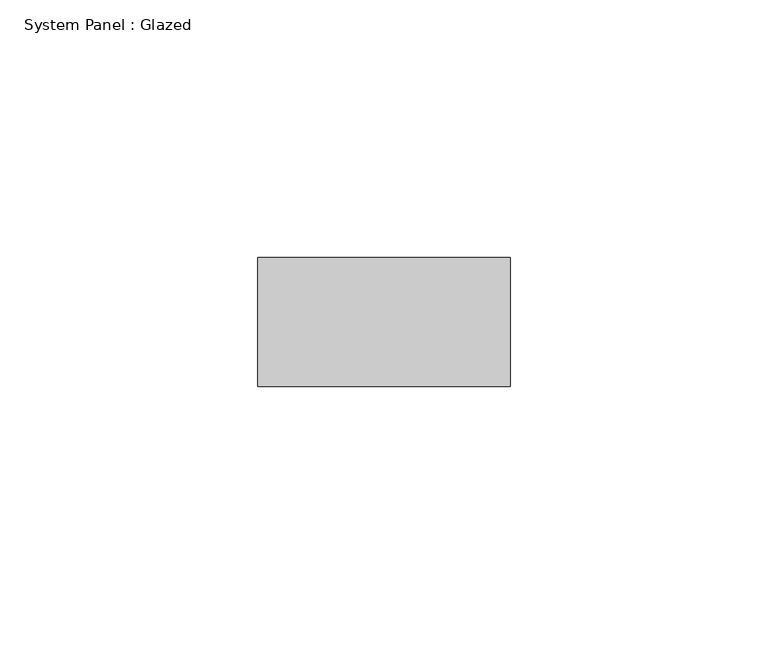
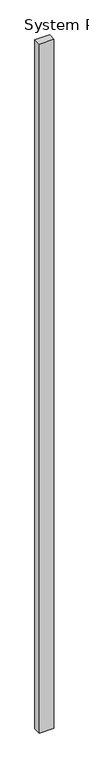
"""IFC4 building model written with IfcOpenShell, lengths in millimetres: plate geometry, System Panel : Glazed."""

import ifcopenshell
import ifcopenshell.guid

model = None  # the IFC model being written
_history = None  # IfcOwnerHistory: only IFC2X3 demands one
_inside = {}  # id of a spatial element -> (the spatial element, [elements in it])
_under = {}  # id of a project, library or spatial element -> (it, [spatial elements below it])
_declared = {}  # id of a project -> (the project, [libraries it declares])
_typed = {}  # id of a type object -> (the type object, [elements of that type])
_made_of = {}  # id of a material, layer set ... -> (it, [elements and type objects made of it])


def new_model(schema):
    """Start an empty IFC model of exactly this schema.

    Asked for "IFC4X3", IfcOpenShell would pick the latest addendum, in which some entities
    have other attributes; the version numbers below select the first issue.
    IFC2X3 requires an IfcOwnerHistory on every rooted entity: one is made here for all.
    """
    global model, _history
    if schema == "IFC4X3":
        model = ifcopenshell.file(schema_version=(4, 3, 0, 0))
    else:
        model = ifcopenshell.file(schema=schema)
    _inside.clear()
    _under.clear()
    _declared.clear()
    _typed.clear()
    _made_of.clear()
    _history = None
    if model.schema == "IFC2X3":
        org = make("IfcOrganization", Name="unknown")
        user = make(
            "IfcPersonAndOrganization",
            ThePerson=make("IfcPerson", FamilyName="unknown"),
            TheOrganization=org,
        )
        app = make(
            "IfcApplication",
            ApplicationDeveloper=org,
            Version="unknown",
            ApplicationFullName="unknown",
            ApplicationIdentifier="unknown",
        )
        _history = make(
            "IfcOwnerHistory",
            OwningUser=user,
            OwningApplication=app,
            ChangeAction="ADDED",
            CreationDate=0,
        )
    return model


def make(cls, **values):
    """One entity of the class cls with the attributes given. An attribute that is None is left unset."""
    return model.create_entity(
        cls, **{name: value for name, value in values.items() if value is not None}
    )


def rooted(cls, **values):
    """An entity with a GlobalId (a new one), such as an element, a storey or a relation."""
    return make(cls, GlobalId=ifcopenshell.guid.new(), OwnerHistory=_history, **values)


def si_unit(unit_type, name, prefix=None):
    """IfcSIUnit, for example si_unit("LENGTHUNIT", "METRE", prefix="MILLI")."""
    return make("IfcSIUnit", UnitType=unit_type, Prefix=prefix, Name=name)


def assignment(units):
    """IfcUnitAssignment: the units of a project."""
    return None if units is None else make("IfcUnitAssignment", Units=units)


def point(xyz):
    """IfcCartesianPoint."""
    return None if xyz is None else make("IfcCartesianPoint", Coordinates=xyz)


def direction(xyz):
    """IfcDirection."""
    return None if xyz is None else make("IfcDirection", DirectionRatios=xyz)


def frame(location, z_axis=None, x_axis=None):
    """IfcAxis2Placement3D, a coordinate frame: its origin and axes. An axis left out is left unset."""
    return make(
        "IfcAxis2Placement3D",
        Location=point(location),
        Axis=direction(z_axis),
        RefDirection=direction(x_axis),
    )


def origin():
    """The frame at (0, 0, 0) with its axes left unset."""
    return frame((0.0, 0.0, 0.0))


def origin_with_axes():
    """The frame at (0, 0, 0) with the z axis (0, 0, 1) and the x axis (1, 0, 0) written out."""
    return frame((0.0, 0.0, 0.0), z_axis=(0.0, 0.0, 1.0), x_axis=(1.0, 0.0, 0.0))


def place(relative_to, where):
    """IfcLocalPlacement: puts the frame where relative to a parent placement (None: the world)."""
    return make(
        "IfcLocalPlacement", PlacementRelTo=relative_to, RelativePlacement=where
    )


def context(
    kind, dimensions, precision=None, world=None, true_north=None, identifier=None
):
    """IfcGeometricRepresentationContext, for example the 3D "Model" context."""
    return make(
        "IfcGeometricRepresentationContext",
        ContextIdentifier=identifier,
        ContextType=kind,
        CoordinateSpaceDimension=dimensions,
        Precision=precision,
        WorldCoordinateSystem=world,
        TrueNorth=true_north,
    )


def project(units=None, contexts=None):
    """IfcProject with its units and contexts."""
    return rooted(
        "IfcProject",
        Name="project",
        RepresentationContexts=contexts,
        UnitsInContext=assignment(units),
    )


def spatial(cls, under=None, at=None, **own):
    """A site, building, storey or space (cls), placed at a placement, below another one or the project."""
    s = rooted(cls, ObjectPlacement=at, **own)
    if under is not None:
        _under.setdefault(under.id(), (under, []))[1].append(s)
    return s


def polyline(points):
    """IfcPolyline through the points."""
    return make("IfcPolyline", Points=[point(p) for p in points])


def outline(outer, holes=None, kind="AREA"):
    """IfcArbitraryClosedProfileDef: a profile drawn as a closed curve; with holes, ...WithVoids."""
    if holes is None:
        return make("IfcArbitraryClosedProfileDef", ProfileType=kind, OuterCurve=outer)
    return make(
        "IfcArbitraryProfileDefWithVoids",
        ProfileType=kind,
        OuterCurve=outer,
        InnerCurves=holes,
    )


def extrude(swept, where, along, depth):
    """IfcExtrudedAreaSolid: the profile swept, set in the frame where, extruded along a direction by depth."""
    return make(
        "IfcExtrudedAreaSolid",
        SweptArea=swept,
        Position=where,
        ExtrudedDirection=direction(along),
        Depth=depth,
    )


def shape(context_of_items, identifier, shape_type, items):
    """IfcShapeRepresentation: the items that make up one representation, for example the "Body"."""
    return make(
        "IfcShapeRepresentation",
        ContextOfItems=context_of_items,
        RepresentationIdentifier=identifier,
        RepresentationType=shape_type,
        Items=items,
    )


def source(mapping_origin, context_of_items, identifier, shape_type, items):
    """IfcRepresentationMap: a shape defined once, which mapped items show again and again."""
    return make(
        "IfcRepresentationMap",
        MappingOrigin=mapping_origin,
        MappedRepresentation=shape(context_of_items, identifier, shape_type, items),
    )


def transform(
    local_origin,
    x_axis=None,
    y_axis=None,
    z_axis=None,
    scale=None,
    scale2=None,
    scale3=None,
    uniform=True,
):
    """IfcCartesianTransformationOperator3D, or its non-uniform kind. x_axis, y_axis, z_axis: its Axis1, 2, 3."""
    if uniform:
        return make(
            "IfcCartesianTransformationOperator3D",
            Axis1=direction(x_axis),
            Axis2=direction(y_axis),
            LocalOrigin=point(local_origin),
            Scale=scale,
            Axis3=direction(z_axis),
        )
    return make(
        "IfcCartesianTransformationOperator3DnonUniform",
        Axis1=direction(x_axis),
        Axis2=direction(y_axis),
        LocalOrigin=point(local_origin),
        Scale=scale,
        Axis3=direction(z_axis),
        Scale2=scale2,
        Scale3=scale3,
    )


def mapped(mapping_source, mapping_target):
    """IfcMappedItem: shows the shape of a source again, moved by a transform."""
    return make(
        "IfcMappedItem", MappingSource=mapping_source, MappingTarget=mapping_target
    )


def made_of(thing, what):
    """Note that an element or type object is made of a material, layer set ...; save() writes the relation."""
    if what is not None:
        _made_of.setdefault(what.id(), (what, []))[1].append(thing)
    return thing


def element(
    cls,
    number,
    at=None,
    inside=None,
    cuts=None,
    type_object=None,
    material=None,
    context=None,
    identifier="Body",
    shape_type=None,
    held_by="IfcProductDefinitionShape",
    body=None,
    shapes=None,
    **own,
):
    """One element of the class cls, such as IfcWall. Its Tag is "e" and its number.

    at: its placement. inside: the storey or other place that contains it. cuts: it is an
    opening in that element (IfcRelVoidsElement). A single representation is given by context,
    identifier, shape_type and body (its items); several are given by shapes. held_by: the class
    of the entity that holds the representations. save() writes the other relations.
    """
    e = rooted(cls, Tag="e%d" % number, ObjectPlacement=at, **own)
    if body is not None:
        shapes = [shape(context, identifier, shape_type, body)]
    if shapes is not None:
        e.Representation = make(held_by, Representations=shapes)
    if inside is not None:
        _inside.setdefault(inside.id(), (inside, []))[1].append(e)
    if cuts is not None:
        rooted(
            "IfcRelVoidsElement", RelatingBuildingElement=cuts, RelatedOpeningElement=e
        )
    if type_object is not None:
        _typed.setdefault(type_object.id(), (type_object, []))[1].append(e)
    return made_of(e, material)


def aggregate(whole, parts):
    """IfcRelAggregates: a whole, such as a stair, and the parts it consists of."""
    return rooted("IfcRelAggregates", RelatingObject=whole, RelatedObjects=parts)


def save(model, path):
    """Write the relations noted so far, then the file.

    IfcRelAggregates (storeys below a building ...), IfcRelContainedInSpatialStructure (elements
    in a storey), IfcRelDefinesByType, IfcRelAssociatesMaterial and IfcRelDeclares: one each for
    every whole, place, type object, material and project.
    """
    for whole, parts in _under.values():
        aggregate(whole, parts)
    for where, things in _inside.values():
        rooted(
            "IfcRelContainedInSpatialStructure",
            RelatedElements=things,
            RelatingStructure=where,
        )
    for kind, things in _typed.values():
        rooted("IfcRelDefinesByType", RelatedObjects=things, RelatingType=kind)
    for what, things in _made_of.values():
        rooted("IfcRelAssociatesMaterial", RelatedObjects=things, RelatingMaterial=what)
    for by, libraries in _declared.values():
        rooted("IfcRelDeclares", RelatingContext=by, RelatedDefinitions=libraries)
    model.write(path)


def system_panel_glazed_7067f38e(model_context):
    return source(origin(), model_context, "Body", "SweptSolid", [
        extrude(outline(polyline([(24.5092572, -49.5), (-24.5092572, -49.5), (-24.5092572, -24.5), (24.5092572, -24.5), (24.5092572, -49.5)])), origin_with_axes(), (0.0, 0.0, 1.0), 2425.0),
    ])


if __name__ == "__main__":
    model = new_model("IFC4")
    model_context = context("Model", 3, world=origin())
    ifc_project = project(units=[si_unit("LENGTHUNIT", "METRE", prefix="MILLI")], contexts=[model_context])
    site = spatial("IfcSite", under=ifc_project)
    building = spatial("IfcBuilding", under=site)
    placement = place(None, origin())
    system_panel_glazed_shape = system_panel_glazed_7067f38e(model_context)
    element("IfcPlate", 1, ObjectType="System Panel : Glazed", at=placement, inside=building, context=model_context, shape_type="MappedRepresentation", body=[
        mapped(system_panel_glazed_shape, transform((0.0, 0.0, 0.0), x_axis=(1.0, 0.0, 0.0), y_axis=(0.0, 1.0, 0.0), z_axis=(0.0, 0.0, 1.0))),
    ])
    save(model, "model.ifc")

# Revit data of these elements
# Type "System Panel : Glazed"
#   Keynote = "H11"
#   Construction Type Id = "GSP4R"
#   Analytic Construction = "1/8 in Pilkington single glazing"
#   Visual Light Transmittance = 0.9
#   Solar Heat Gain Coefficient = 0.86
#   Heat Transfer Coefficient (U) = 6.7069 W/(m²·K)
# Element 1 (IfcPlate, "System Panel : Glazed")
#   Materials on its faces: "Glass"
# Materials
#   "Glass": class "Glass", colour RGB 0 128 192, transparency 0.9, Description = "Soda Lime Glass", Cost = 0
